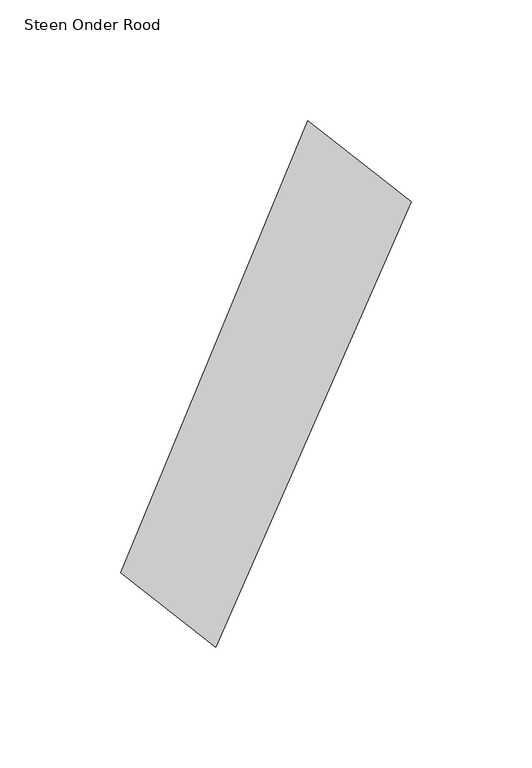
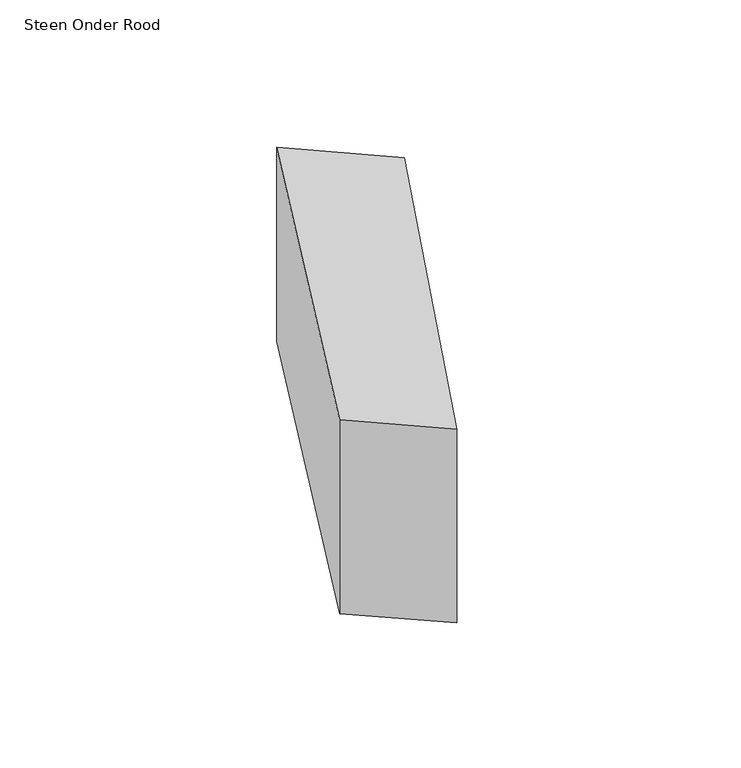
"""IFC4 building model written with IfcOpenShell, lengths in millimetres: proxy geometry, 00_GMA_steen_versie_4 : Steen Onder Rood."""

from ifc_helpers import new_model, si_unit, origin, origin_with_axes, place, context, project, spatial, polyline, outline, extrude, source, transform, mapped, element, save


def steen_onder_rood_8646319a(model_context):
    return source(origin(), model_context, "Body", "SweptSolid", [
        extrude(outline(polyline([(140.9952697, 161.6466832), (60.2245729, -22.8796698), (20.8107144, 7.8863465), (98.1708523, 195.1035769), (140.9952697, 161.6466832)])), origin_with_axes(), (0.0, 0.0, 1.0), 100.0),
    ])


if __name__ == "__main__":
    model = new_model("IFC4")
    model_context = context("Model", 3, world=origin())
    ifc_project = project(units=[si_unit("LENGTHUNIT", "METRE", prefix="MILLI")], contexts=[model_context])
    site = spatial("IfcSite", under=ifc_project)
    building = spatial("IfcBuilding", under=site)
    placement = place(None, origin())
    steen_onder_rood_shape = steen_onder_rood_8646319a(model_context)
    element("IfcBuildingElementProxy", 1, Name="00_GMA_steen_versie_4 : Steen Onder Rood", ObjectType="00_GMA_steen_versie_4 : Steen Onder Rood", at=placement, inside=building, context=model_context, shape_type="MappedRepresentation", body=[
        mapped(steen_onder_rood_shape, transform((0.0, 0.0, 0.0), x_axis=(1.0, 0.0, 0.0), y_axis=(0.0, 1.0, 0.0), z_axis=(0.0, 0.0, 1.0))),
    ])
    save(model, "model.ifc")

# Revit data of these elements
# Type "00_GMA_steen_versie_4 : Steen Onder Rood"
#   StootVoegHalfBoven [instance default] = 5 mm
#   StootVoegHalf [instance default] = 5 mm
#   StootVoegBreedteOnder = 10 mm
#   StootVoegBreedteBoven = 10 mm
#   Steendikte = 100 mm
#   LintVoegOnderHalf = 0 mm
#   LintVoegOnder = 0 mm
#   LintVoegBovenHalf = 5 mm
#   LintVoegBoven = 10 mm
#   materiaal = 21_steen_rood
#   MateriaalVoeg = none
#   Default Elevation = 0
# Element 1 (IfcBuildingElementProxy, "00_GMA_steen_versie_4 : Steen Onder Rood")
#   Materials on its faces: "21_steen_rood"
# Materials
#   "21_steen_rood": class "Unassigned", colour RGB 213 111 43, transparency 0, Cost = 0
